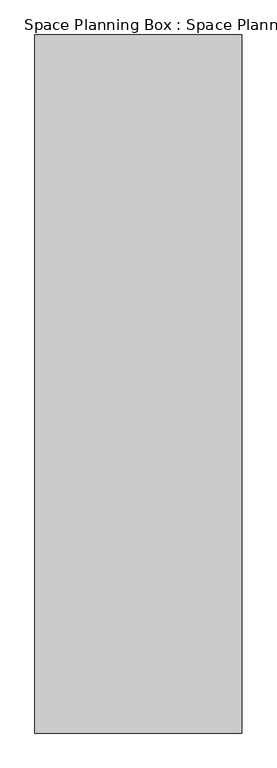
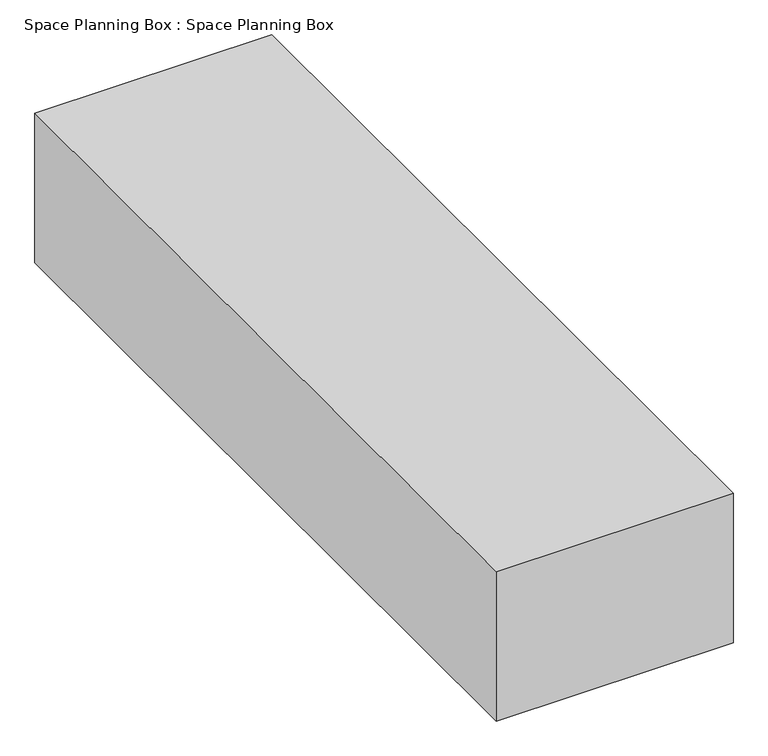
"""IFC4 building model written with IfcOpenShell, lengths in millimetres: proxy geometry, Space Planning Box : Space Planning Box."""

import ifcopenshell
import ifcopenshell.guid

model = None  # the IFC model being written
_history = None  # IfcOwnerHistory: only IFC2X3 demands one
_inside = {}  # id of a spatial element -> (the spatial element, [elements in it])
_under = {}  # id of a project, library or spatial element -> (it, [spatial elements below it])
_declared = {}  # id of a project -> (the project, [libraries it declares])
_typed = {}  # id of a type object -> (the type object, [elements of that type])
_made_of = {}  # id of a material, layer set ... -> (it, [elements and type objects made of it])


def new_model(schema):
    """Start an empty IFC model of exactly this schema.

    Asked for "IFC4X3", IfcOpenShell would pick the latest addendum, in which some entities
    have other attributes; the version numbers below select the first issue.
    IFC2X3 requires an IfcOwnerHistory on every rooted entity: one is made here for all.
    """
    global model, _history
    if schema == "IFC4X3":
        model = ifcopenshell.file(schema_version=(4, 3, 0, 0))
    else:
        model = ifcopenshell.file(schema=schema)
    _inside.clear()
    _under.clear()
    _declared.clear()
    _typed.clear()
    _made_of.clear()
    _history = None
    if model.schema == "IFC2X3":
        org = make("IfcOrganization", Name="unknown")
        user = make(
            "IfcPersonAndOrganization",
            ThePerson=make("IfcPerson", FamilyName="unknown"),
            TheOrganization=org,
        )
        app = make(
            "IfcApplication",
            ApplicationDeveloper=org,
            Version="unknown",
            ApplicationFullName="unknown",
            ApplicationIdentifier="unknown",
        )
        _history = make(
            "IfcOwnerHistory",
            OwningUser=user,
            OwningApplication=app,
            ChangeAction="ADDED",
            CreationDate=0,
        )
    return model


def make(cls, **values):
    """One entity of the class cls with the attributes given. An attribute that is None is left unset."""
    return model.create_entity(
        cls, **{name: value for name, value in values.items() if value is not None}
    )


def rooted(cls, **values):
    """An entity with a GlobalId (a new one), such as an element, a storey or a relation."""
    return make(cls, GlobalId=ifcopenshell.guid.new(), OwnerHistory=_history, **values)


def si_unit(unit_type, name, prefix=None):
    """IfcSIUnit, for example si_unit("LENGTHUNIT", "METRE", prefix="MILLI")."""
    return make("IfcSIUnit", UnitType=unit_type, Prefix=prefix, Name=name)


def assignment(units):
    """IfcUnitAssignment: the units of a project."""
    return None if units is None else make("IfcUnitAssignment", Units=units)


def point(xyz):
    """IfcCartesianPoint."""
    return None if xyz is None else make("IfcCartesianPoint", Coordinates=xyz)


def direction(xyz):
    """IfcDirection."""
    return None if xyz is None else make("IfcDirection", DirectionRatios=xyz)


def frame(location, z_axis=None, x_axis=None):
    """IfcAxis2Placement3D, a coordinate frame: its origin and axes. An axis left out is left unset."""
    return make(
        "IfcAxis2Placement3D",
        Location=point(location),
        Axis=direction(z_axis),
        RefDirection=direction(x_axis),
    )


def origin():
    """The frame at (0, 0, 0) with its axes left unset."""
    return frame((0.0, 0.0, 0.0))


def origin_with_axes():
    """The frame at (0, 0, 0) with the z axis (0, 0, 1) and the x axis (1, 0, 0) written out."""
    return frame((0.0, 0.0, 0.0), z_axis=(0.0, 0.0, 1.0), x_axis=(1.0, 0.0, 0.0))


def place(relative_to, where):
    """IfcLocalPlacement: puts the frame where relative to a parent placement (None: the world)."""
    return make(
        "IfcLocalPlacement", PlacementRelTo=relative_to, RelativePlacement=where
    )


def context(
    kind, dimensions, precision=None, world=None, true_north=None, identifier=None
):
    """IfcGeometricRepresentationContext, for example the 3D "Model" context."""
    return make(
        "IfcGeometricRepresentationContext",
        ContextIdentifier=identifier,
        ContextType=kind,
        CoordinateSpaceDimension=dimensions,
        Precision=precision,
        WorldCoordinateSystem=world,
        TrueNorth=true_north,
    )


def project(units=None, contexts=None):
    """IfcProject with its units and contexts."""
    return rooted(
        "IfcProject",
        Name="project",
        RepresentationContexts=contexts,
        UnitsInContext=assignment(units),
    )


def spatial(cls, under=None, at=None, **own):
    """A site, building, storey or space (cls), placed at a placement, below another one or the project."""
    s = rooted(cls, ObjectPlacement=at, **own)
    if under is not None:
        _under.setdefault(under.id(), (under, []))[1].append(s)
    return s


def polyline(points):
    """IfcPolyline through the points."""
    return make("IfcPolyline", Points=[point(p) for p in points])


def outline(outer, holes=None, kind="AREA"):
    """IfcArbitraryClosedProfileDef: a profile drawn as a closed curve; with holes, ...WithVoids."""
    if holes is None:
        return make("IfcArbitraryClosedProfileDef", ProfileType=kind, OuterCurve=outer)
    return make(
        "IfcArbitraryProfileDefWithVoids",
        ProfileType=kind,
        OuterCurve=outer,
        InnerCurves=holes,
    )


def extrude(swept, where, along, depth):
    """IfcExtrudedAreaSolid: the profile swept, set in the frame where, extruded along a direction by depth."""
    return make(
        "IfcExtrudedAreaSolid",
        SweptArea=swept,
        Position=where,
        ExtrudedDirection=direction(along),
        Depth=depth,
    )


def shape(context_of_items, identifier, shape_type, items):
    """IfcShapeRepresentation: the items that make up one representation, for example the "Body"."""
    return make(
        "IfcShapeRepresentation",
        ContextOfItems=context_of_items,
        RepresentationIdentifier=identifier,
        RepresentationType=shape_type,
        Items=items,
    )


def source(mapping_origin, context_of_items, identifier, shape_type, items):
    """IfcRepresentationMap: a shape defined once, which mapped items show again and again."""
    return make(
        "IfcRepresentationMap",
        MappingOrigin=mapping_origin,
        MappedRepresentation=shape(context_of_items, identifier, shape_type, items),
    )


def transform(
    local_origin,
    x_axis=None,
    y_axis=None,
    z_axis=None,
    scale=None,
    scale2=None,
    scale3=None,
    uniform=True,
):
    """IfcCartesianTransformationOperator3D, or its non-uniform kind. x_axis, y_axis, z_axis: its Axis1, 2, 3."""
    if uniform:
        return make(
            "IfcCartesianTransformationOperator3D",
            Axis1=direction(x_axis),
            Axis2=direction(y_axis),
            LocalOrigin=point(local_origin),
            Scale=scale,
            Axis3=direction(z_axis),
        )
    return make(
        "IfcCartesianTransformationOperator3DnonUniform",
        Axis1=direction(x_axis),
        Axis2=direction(y_axis),
        LocalOrigin=point(local_origin),
        Scale=scale,
        Axis3=direction(z_axis),
        Scale2=scale2,
        Scale3=scale3,
    )


def mapped(mapping_source, mapping_target):
    """IfcMappedItem: shows the shape of a source again, moved by a transform."""
    return make(
        "IfcMappedItem", MappingSource=mapping_source, MappingTarget=mapping_target
    )


def made_of(thing, what):
    """Note that an element or type object is made of a material, layer set ...; save() writes the relation."""
    if what is not None:
        _made_of.setdefault(what.id(), (what, []))[1].append(thing)
    return thing


def element(
    cls,
    number,
    at=None,
    inside=None,
    cuts=None,
    type_object=None,
    material=None,
    context=None,
    identifier="Body",
    shape_type=None,
    held_by="IfcProductDefinitionShape",
    body=None,
    shapes=None,
    **own,
):
    """One element of the class cls, such as IfcWall. Its Tag is "e" and its number.

    at: its placement. inside: the storey or other place that contains it. cuts: it is an
    opening in that element (IfcRelVoidsElement). A single representation is given by context,
    identifier, shape_type and body (its items); several are given by shapes. held_by: the class
    of the entity that holds the representations. save() writes the other relations.
    """
    e = rooted(cls, Tag="e%d" % number, ObjectPlacement=at, **own)
    if body is not None:
        shapes = [shape(context, identifier, shape_type, body)]
    if shapes is not None:
        e.Representation = make(held_by, Representations=shapes)
    if inside is not None:
        _inside.setdefault(inside.id(), (inside, []))[1].append(e)
    if cuts is not None:
        rooted(
            "IfcRelVoidsElement", RelatingBuildingElement=cuts, RelatedOpeningElement=e
        )
    if type_object is not None:
        _typed.setdefault(type_object.id(), (type_object, []))[1].append(e)
    return made_of(e, material)


def aggregate(whole, parts):
    """IfcRelAggregates: a whole, such as a stair, and the parts it consists of."""
    return rooted("IfcRelAggregates", RelatingObject=whole, RelatedObjects=parts)


def save(model, path):
    """Write the relations noted so far, then the file.

    IfcRelAggregates (storeys below a building ...), IfcRelContainedInSpatialStructure (elements
    in a storey), IfcRelDefinesByType, IfcRelAssociatesMaterial and IfcRelDeclares: one each for
    every whole, place, type object, material and project.
    """
    for whole, parts in _under.values():
        aggregate(whole, parts)
    for where, things in _inside.values():
        rooted(
            "IfcRelContainedInSpatialStructure",
            RelatedElements=things,
            RelatingStructure=where,
        )
    for kind, things in _typed.values():
        rooted("IfcRelDefinesByType", RelatedObjects=things, RelatingType=kind)
    for what, things in _made_of.values():
        rooted("IfcRelAssociatesMaterial", RelatedObjects=things, RelatingMaterial=what)
    for by, libraries in _declared.values():
        rooted("IfcRelDeclares", RelatingContext=by, RelatedDefinitions=libraries)
    model.write(path)


def space_planning_box_space_planning_box_ce7d2093(model_context):
    return source(origin(), model_context, "Body", "SweptSolid", [
        extrude(outline(polyline([(4500.0, 15175.0), (4500.0, -15175.0), (-4500.0, -15175.0), (-4500.0, 15175.0), (4500.0, 15175.0)])), origin_with_axes(), (0.0, 0.0, 1.0), 6000.0),
    ])


if __name__ == "__main__":
    model = new_model("IFC4")
    model_context = context("Model", 3, world=origin())
    ifc_project = project(units=[si_unit("LENGTHUNIT", "METRE", prefix="MILLI")], contexts=[model_context])
    site = spatial("IfcSite", under=ifc_project)
    building = spatial("IfcBuilding", under=site)
    placement = place(None, origin())
    space_planning_box_space_planning_box_shape = space_planning_box_space_planning_box_ce7d2093(model_context)
    element("IfcBuildingElementProxy", 1, Name="Space Planning Box : Space Planning Box", ObjectType="Space Planning Box : Space Planning Box", at=placement, inside=building, context=model_context, shape_type="MappedRepresentation", body=[
        mapped(space_planning_box_space_planning_box_shape, transform((0.0, 0.0, 0.0), x_axis=(1.0, 0.0, 0.0), y_axis=(0.0, 1.0, 0.0), z_axis=(0.0, 0.0, 1.0))),
    ])
    save(model, "model.ifc")

# Revit data of these elements
# Type "Space Planning Box : Space Planning Box"
#   Type Comments = "..."
#   Room Name [instance default] = "?"
#   Assembly Code = "..."
#   Width [instance default] = 1524 mm
#   Program Area [instance default] = 0 m²
#   Length [instance default] = 1524 mm
#   Height [instance default] = 1524 mm
#   Area [instance default] = 2.32258 m²
#   Fill Color [instance default] = Cyan
#   Default Elevation = 0
# Element 1 (IfcBuildingElementProxy, "Space Planning Box : Space Planning Box")
#   Room Name = "Central Control Room"
#   Width = 9000 mm
#   Program Area = 288 m²
#   Length = 30350 mm
#   Height = 6000 mm
#   Area = 273.15 m²
#   Fill Color = Lime
#   Materials on its faces: "Lime"
# Materials
#   "Cyan": class "Generic", colour RGB 0 255 255, transparency 0.2, Cost = 0
#   "Lime": class "Generic", colour RGB 0 255 0, transparency 0.2, Cost = 0
